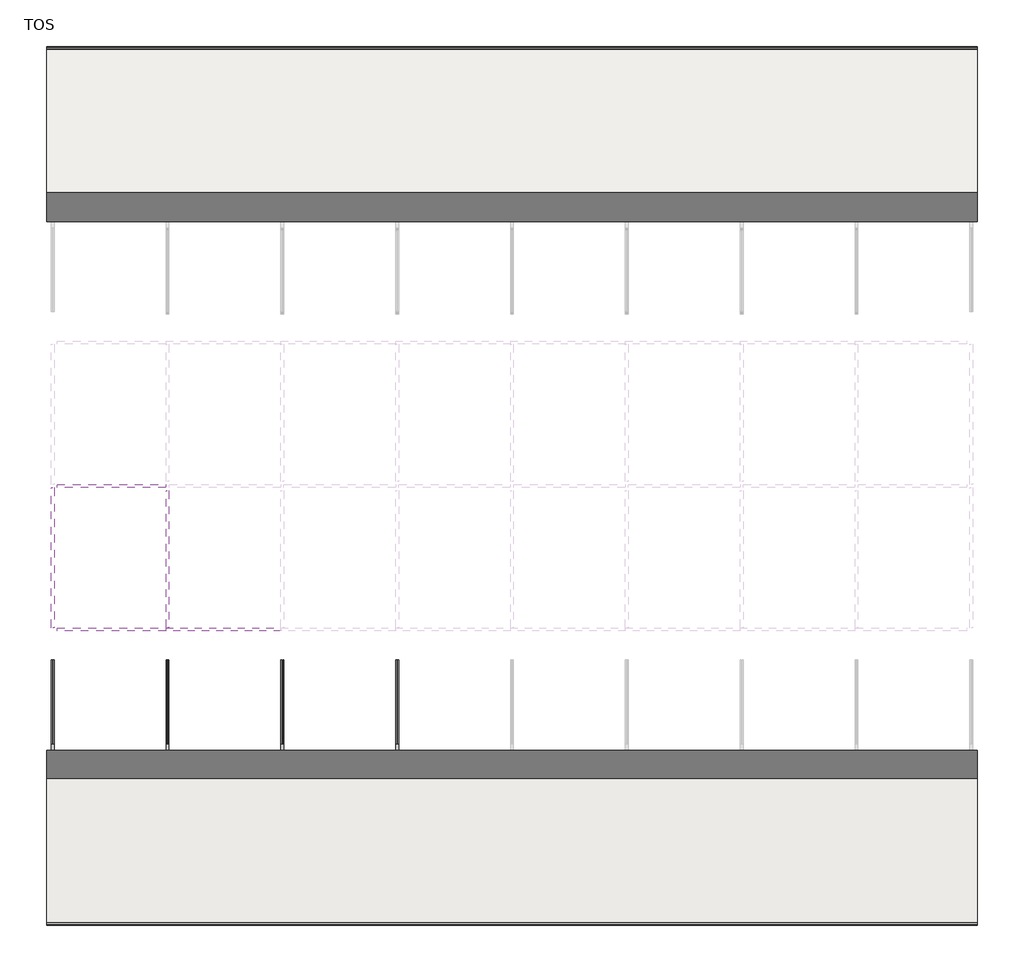
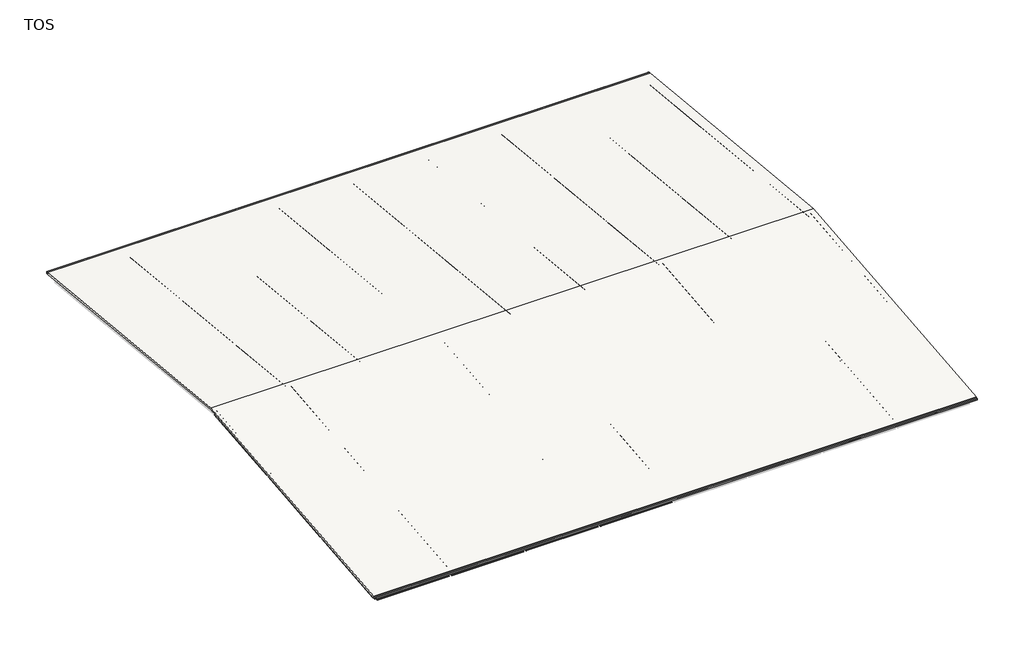
# One storey, part 1 of 5: 21 beams, 1 pipe segment, 1 roof.
"""IFC4 building model written with IfcOpenShell, lengths in millimetres."""

import ifcopenshell
import ifcopenshell.guid

model = None  # the IFC model being written
_history = None  # IfcOwnerHistory: only IFC2X3 demands one
_inside = {}  # id of a spatial element -> (the spatial element, [elements in it])
_under = {}  # id of a project, library or spatial element -> (it, [spatial elements below it])
_declared = {}  # id of a project -> (the project, [libraries it declares])
_typed = {}  # id of a type object -> (the type object, [elements of that type])
_made_of = {}  # id of a material, layer set ... -> (it, [elements and type objects made of it])


def new_model(schema):
    """Start an empty IFC model of exactly this schema.

    Asked for "IFC4X3", IfcOpenShell would pick the latest addendum, in which some entities
    have other attributes; the version numbers below select the first issue.
    IFC2X3 requires an IfcOwnerHistory on every rooted entity: one is made here for all.
    """
    global model, _history
    if schema == "IFC4X3":
        model = ifcopenshell.file(schema_version=(4, 3, 0, 0))
    else:
        model = ifcopenshell.file(schema=schema)
    _inside.clear()
    _under.clear()
    _declared.clear()
    _typed.clear()
    _made_of.clear()
    _history = None
    if model.schema == "IFC2X3":
        org = make("IfcOrganization", Name="unknown")
        user = make(
            "IfcPersonAndOrganization",
            ThePerson=make("IfcPerson", FamilyName="unknown"),
            TheOrganization=org,
        )
        app = make(
            "IfcApplication",
            ApplicationDeveloper=org,
            Version="unknown",
            ApplicationFullName="unknown",
            ApplicationIdentifier="unknown",
        )
        _history = make(
            "IfcOwnerHistory",
            OwningUser=user,
            OwningApplication=app,
            ChangeAction="ADDED",
            CreationDate=0,
        )
    return model


def make(cls, **values):
    """One entity of the class cls with the attributes given. An attribute that is None is left unset."""
    return model.create_entity(
        cls, **{name: value for name, value in values.items() if value is not None}
    )


def rooted(cls, **values):
    """An entity with a GlobalId (a new one), such as an element, a storey or a relation."""
    return make(cls, GlobalId=ifcopenshell.guid.new(), OwnerHistory=_history, **values)


def si_unit(unit_type, name, prefix=None):
    """IfcSIUnit, for example si_unit("LENGTHUNIT", "METRE", prefix="MILLI")."""
    return make("IfcSIUnit", UnitType=unit_type, Prefix=prefix, Name=name)


def assignment(units):
    """IfcUnitAssignment: the units of a project."""
    return None if units is None else make("IfcUnitAssignment", Units=units)


def point(xyz):
    """IfcCartesianPoint."""
    return None if xyz is None else make("IfcCartesianPoint", Coordinates=xyz)


def direction(xyz):
    """IfcDirection."""
    return None if xyz is None else make("IfcDirection", DirectionRatios=xyz)


def frame(location, z_axis=None, x_axis=None):
    """IfcAxis2Placement3D, a coordinate frame: its origin and axes. An axis left out is left unset."""
    return make(
        "IfcAxis2Placement3D",
        Location=point(location),
        Axis=direction(z_axis),
        RefDirection=direction(x_axis),
    )


def frame_2d(location, x_axis=None):
    """IfcAxis2Placement2D, a coordinate frame in the plane: its origin and x axis."""
    return make(
        "IfcAxis2Placement2D", Location=point(location), RefDirection=direction(x_axis)
    )


def origin():
    """The frame at (0, 0, 0) with its axes left unset."""
    return frame((0.0, 0.0, 0.0))


def place(relative_to, where):
    """IfcLocalPlacement: puts the frame where relative to a parent placement (None: the world)."""
    return make(
        "IfcLocalPlacement", PlacementRelTo=relative_to, RelativePlacement=where
    )


def context(
    kind, dimensions, precision=None, world=None, true_north=None, identifier=None
):
    """IfcGeometricRepresentationContext, for example the 3D "Model" context."""
    return make(
        "IfcGeometricRepresentationContext",
        ContextIdentifier=identifier,
        ContextType=kind,
        CoordinateSpaceDimension=dimensions,
        Precision=precision,
        WorldCoordinateSystem=world,
        TrueNorth=true_north,
    )


def project(units=None, contexts=None):
    """IfcProject with its units and contexts."""
    return rooted(
        "IfcProject",
        Name="project",
        RepresentationContexts=contexts,
        UnitsInContext=assignment(units),
    )


def spatial(cls, under=None, at=None, **own):
    """A site, building, storey or space (cls), placed at a placement, below another one or the project."""
    s = rooted(cls, ObjectPlacement=at, **own)
    if under is not None:
        _under.setdefault(under.id(), (under, []))[1].append(s)
    return s


def polyline(points):
    """IfcPolyline through the points."""
    return make("IfcPolyline", Points=[point(p) for p in points])


def circle_curve(where, radius):
    """IfcCircle in the frame where."""
    return make("IfcCircle", Position=where, Radius=radius)


def trimmed(basis, trim1, trim2, sense, master):
    """IfcTrimmedCurve: the piece of a basis curve between two trims."""
    return make(
        "IfcTrimmedCurve",
        BasisCurve=basis,
        Trim1=trim1,
        Trim2=trim2,
        SenseAgreement=sense,
        MasterRepresentation=master,
    )


def segment(curve, same_sense, transition):
    """IfcCompositeCurveSegment."""
    return make(
        "IfcCompositeCurveSegment",
        Transition=transition,
        SameSense=same_sense,
        ParentCurve=curve,
    )


def composite_curve(segments, self_intersect=None):
    """IfcCompositeCurve: segments joined end to end."""
    return make("IfcCompositeCurve", Segments=segments, SelfIntersect=self_intersect)


def outline(outer, holes=None, kind="AREA"):
    """IfcArbitraryClosedProfileDef: a profile drawn as a closed curve; with holes, ...WithVoids."""
    if holes is None:
        return make("IfcArbitraryClosedProfileDef", ProfileType=kind, OuterCurve=outer)
    return make(
        "IfcArbitraryProfileDefWithVoids",
        ProfileType=kind,
        OuterCurve=outer,
        InnerCurves=holes,
    )


def extrude(swept, where, along, depth):
    """IfcExtrudedAreaSolid: the profile swept, set in the frame where, extruded along a direction by depth."""
    return make(
        "IfcExtrudedAreaSolid",
        SweptArea=swept,
        Position=where,
        ExtrudedDirection=direction(along),
        Depth=depth,
    )


def shape(context_of_items, identifier, shape_type, items):
    """IfcShapeRepresentation: the items that make up one representation, for example the "Body"."""
    return make(
        "IfcShapeRepresentation",
        ContextOfItems=context_of_items,
        RepresentationIdentifier=identifier,
        RepresentationType=shape_type,
        Items=items,
    )


def made_of(thing, what):
    """Note that an element or type object is made of a material, layer set ...; save() writes the relation."""
    if what is not None:
        _made_of.setdefault(what.id(), (what, []))[1].append(thing)
    return thing


def element(
    cls,
    number,
    at=None,
    inside=None,
    cuts=None,
    type_object=None,
    material=None,
    context=None,
    identifier="Body",
    shape_type=None,
    held_by="IfcProductDefinitionShape",
    body=None,
    shapes=None,
    **own,
):
    """One element of the class cls, such as IfcWall. Its Tag is "e" and its number.

    at: its placement. inside: the storey or other place that contains it. cuts: it is an
    opening in that element (IfcRelVoidsElement). A single representation is given by context,
    identifier, shape_type and body (its items); several are given by shapes. held_by: the class
    of the entity that holds the representations. save() writes the other relations.
    """
    e = rooted(cls, Tag="e%d" % number, ObjectPlacement=at, **own)
    if body is not None:
        shapes = [shape(context, identifier, shape_type, body)]
    if shapes is not None:
        e.Representation = make(held_by, Representations=shapes)
    if inside is not None:
        _inside.setdefault(inside.id(), (inside, []))[1].append(e)
    if cuts is not None:
        rooted(
            "IfcRelVoidsElement", RelatingBuildingElement=cuts, RelatedOpeningElement=e
        )
    if type_object is not None:
        _typed.setdefault(type_object.id(), (type_object, []))[1].append(e)
    return made_of(e, material)


def aggregate(whole, parts):
    """IfcRelAggregates: a whole, such as a stair, and the parts it consists of."""
    return rooted("IfcRelAggregates", RelatingObject=whole, RelatedObjects=parts)


def save(model, path):
    """Write the relations noted so far, then the file.

    IfcRelAggregates (storeys below a building ...), IfcRelContainedInSpatialStructure (elements
    in a storey), IfcRelDefinesByType, IfcRelAssociatesMaterial and IfcRelDeclares: one each for
    every whole, place, type object, material and project.
    """
    for whole, parts in _under.values():
        aggregate(whole, parts)
    for where, things in _inside.values():
        rooted(
            "IfcRelContainedInSpatialStructure",
            RelatedElements=things,
            RelatingStructure=where,
        )
    for kind, things in _typed.values():
        rooted("IfcRelDefinesByType", RelatedObjects=things, RelatingType=kind)
    for what, things in _made_of.values():
        rooted("IfcRelAssociatesMaterial", RelatedObjects=things, RelatingMaterial=what)
    for by, libraries in _declared.values():
        rooted("IfcRelDeclares", RelatingContext=by, RelatedDefinitions=libraries)
    model.write(path)


model = new_model("IFC4")

# Units and contexts
model_context = context("Model", 3, world=origin())
ifc_project = project(units=[si_unit("LENGTHUNIT", "METRE", prefix="MILLI")], contexts=[model_context])

# Site, building, storey
site = spatial("IfcSite", under=ifc_project)
building = spatial("IfcBuilding", under=site)
storey = spatial("IfcBuildingStorey", under=building, Name="TOS", Elevation=9299.9618634)

# Beams
placement = place(None, origin())
element("IfcBeam", 1, ObjectType="0912_Steel Framing_H-KSD3502 : H_SB_ASB_H-600x200x11x17", at=placement, inside=storey, context=model_context, shape_type="SweptSolid", body=[
    extrude(outline(composite_curve([segment(polyline([(10599.5208589, 9716.9618634), (10599.5208589, 9699.9618634), (10399.5208589, 9699.9618634), (10399.5208589, 9716.9618634), (10472.0208589, 9716.9618634)]), True, "CONTINUOUS"), segment(trimmed(circle_curve(frame_2d((10472.0208589, 9738.9618634)), 22.0), [point((10472.0208589, 9716.9618634))], [point((10494.0208589, 9738.9618634))], True, "CARTESIAN"), True, "CONTINUOUS"), segment(polyline([(10494.0208589, 9738.9618634), (10494.0208589, 10260.9618634)]), True, "CONTINUOUS"), segment(trimmed(circle_curve(frame_2d((10472.0208589, 10260.9618634)), 22.0), [point((10494.0208589, 10260.9618634))], [point((10472.0208589, 10282.9618634))], True, "CARTESIAN"), True, "CONTINUOUS"), segment(polyline([(10472.0208589, 10282.9618634), (10399.5208589, 10282.9618634), (10399.5208589, 10299.9618634), (10599.5208589, 10299.9618634), (10599.5208589, 10282.9618634), (10527.0208589, 10282.9618634)]), True, "CONTINUOUS"), segment(trimmed(circle_curve(frame_2d((10527.0208589, 10260.9618634)), 22.0), [point((10527.0208589, 10282.9618634))], [point((10505.0208589, 10260.9618634))], True, "CARTESIAN"), True, "CONTINUOUS"), segment(polyline([(10505.0208589, 10260.9618634), (10505.0208589, 9738.9618634)]), True, "CONTINUOUS"), segment(trimmed(circle_curve(frame_2d((10527.0208589, 9738.9618634)), 22.0), [point((10505.0208589, 9738.9618634))], [point((10527.0208589, 9716.9618634))], True, "CARTESIAN"), True, "CONTINUOUS"), segment(polyline([(10527.0208589, 9716.9618634), (10599.5208589, 9716.9618634)]), True, "CONTINUOUS")], self_intersect=False)), frame((318.7, 0.0, 0.0), z_axis=(1.0, 0.0, 0.0), x_axis=(0.0, 1.0, 0.0)), (0.0, 0.0, 1.0), 7568.6),
])
element("IfcBeam", 2, ObjectType="0912_Steel Framing_H-KSD3502 : H_SB_ASB_H-600x200x11x17", at=placement, inside=storey, context=model_context, shape_type="SweptSolid", body=[
    extrude(outline(composite_curve([segment(polyline([(10599.5208589, 9716.9618634), (10599.5208589, 9699.9618634), (10399.5208589, 9699.9618634), (10399.5208589, 9716.9618634), (10472.0208589, 9716.9618634)]), True, "CONTINUOUS"), segment(trimmed(circle_curve(frame_2d((10472.0208589, 9738.9618634)), 22.0), [point((10472.0208589, 9716.9618634))], [point((10494.0208589, 9738.9618634))], True, "CARTESIAN"), True, "CONTINUOUS"), segment(polyline([(10494.0208589, 9738.9618634), (10494.0208589, 10260.9618634)]), True, "CONTINUOUS"), segment(trimmed(circle_curve(frame_2d((10472.0208589, 10260.9618634)), 22.0), [point((10494.0208589, 10260.9618634))], [point((10472.0208589, 10282.9618634))], True, "CARTESIAN"), True, "CONTINUOUS"), segment(polyline([(10472.0208589, 10282.9618634), (10399.5208589, 10282.9618634), (10399.5208589, 10299.9618634), (10599.5208589, 10299.9618634), (10599.5208589, 10282.9618634), (10527.0208589, 10282.9618634)]), True, "CONTINUOUS"), segment(trimmed(circle_curve(frame_2d((10527.0208589, 10260.9618634)), 22.0), [point((10527.0208589, 10282.9618634))], [point((10505.0208589, 10260.9618634))], True, "CARTESIAN"), True, "CONTINUOUS"), segment(polyline([(10505.0208589, 10260.9618634), (10505.0208589, 9738.9618634)]), True, "CONTINUOUS"), segment(trimmed(circle_curve(frame_2d((10527.0208589, 9738.9618634)), 22.0), [point((10505.0208589, 9738.9618634))], [point((10527.0208589, 9716.9618634))], True, "CARTESIAN"), True, "CONTINUOUS"), segment(polyline([(10527.0208589, 9716.9618634), (10599.5208589, 9716.9618634)]), True, "CONTINUOUS")], self_intersect=False)), frame((7900.0, 0.0, 0.0), z_axis=(1.0, 0.0, 0.0), x_axis=(0.0, 1.0, 0.0)), (0.0, 0.0, 1.0), 7987.3),
])
element("IfcBeam", 3, ObjectType="0912_Steel Framing_H-KSD3502 : H_SB_ASB_H-600x200x11x17", at=placement, inside=storey, context=model_context, shape_type="SweptSolid", body=[
    extrude(outline(composite_curve([segment(polyline([(10599.5208589, 9716.9618634), (10599.5208589, 9699.9618634), (10399.5208589, 9699.9618634), (10399.5208589, 9716.9618634), (10472.0208589, 9716.9618634)]), True, "CONTINUOUS"), segment(trimmed(circle_curve(frame_2d((10472.0208589, 9738.9618634)), 22.0), [point((10472.0208589, 9716.9618634))], [point((10494.0208589, 9738.9618634))], True, "CARTESIAN"), True, "CONTINUOUS"), segment(polyline([(10494.0208589, 9738.9618634), (10494.0208589, 10260.9618634)]), True, "CONTINUOUS"), segment(trimmed(circle_curve(frame_2d((10472.0208589, 10260.9618634)), 22.0), [point((10494.0208589, 10260.9618634))], [point((10472.0208589, 10282.9618634))], True, "CARTESIAN"), True, "CONTINUOUS"), segment(polyline([(10472.0208589, 10282.9618634), (10399.5208589, 10282.9618634), (10399.5208589, 10299.9618634), (10599.5208589, 10299.9618634), (10599.5208589, 10282.9618634), (10527.0208589, 10282.9618634)]), True, "CONTINUOUS"), segment(trimmed(circle_curve(frame_2d((10527.0208589, 10260.9618634)), 22.0), [point((10527.0208589, 10282.9618634))], [point((10505.0208589, 10260.9618634))], True, "CARTESIAN"), True, "CONTINUOUS"), segment(polyline([(10505.0208589, 10260.9618634), (10505.0208589, 9738.9618634)]), True, "CONTINUOUS"), segment(trimmed(circle_curve(frame_2d((10527.0208589, 9738.9618634)), 22.0), [point((10505.0208589, 9738.9618634))], [point((10527.0208589, 9716.9618634))], True, "CARTESIAN"), True, "CONTINUOUS"), segment(polyline([(10527.0208589, 9716.9618634), (10599.5208589, 9716.9618634)]), True, "CONTINUOUS")], self_intersect=False)), frame((15900.0, 0.0, 0.0), z_axis=(1.0, 0.0, 0.0), x_axis=(0.0, 1.0, 0.0)), (0.0, 0.0, 1.0), 7987.3),
])
element("IfcBeam", 4, ObjectType="0912_Steel Framing_H-KSD3502 : H_SB_ASB_H-600x200x11x17", at=placement, inside=storey, context=model_context, shape_type="SweptSolid", body=[
    extrude(outline(composite_curve([segment(polyline([(10599.5208589, 9716.9618634), (10599.5208589, 9699.9618634), (10399.5208589, 9699.9618634), (10399.5208589, 9716.9618634), (10472.0208589, 9716.9618634)]), True, "CONTINUOUS"), segment(trimmed(circle_curve(frame_2d((10472.0208589, 9738.9618634)), 22.0), [point((10472.0208589, 9716.9618634))], [point((10494.0208589, 9738.9618634))], True, "CARTESIAN"), True, "CONTINUOUS"), segment(polyline([(10494.0208589, 9738.9618634), (10494.0208589, 10260.9618634)]), True, "CONTINUOUS"), segment(trimmed(circle_curve(frame_2d((10472.0208589, 10260.9618634)), 22.0), [point((10494.0208589, 10260.9618634))], [point((10472.0208589, 10282.9618634))], True, "CARTESIAN"), True, "CONTINUOUS"), segment(polyline([(10472.0208589, 10282.9618634), (10399.5208589, 10282.9618634), (10399.5208589, 10299.9618634), (10599.5208589, 10299.9618634), (10599.5208589, 10282.9618634), (10527.0208589, 10282.9618634)]), True, "CONTINUOUS"), segment(trimmed(circle_curve(frame_2d((10527.0208589, 10260.9618634)), 22.0), [point((10527.0208589, 10282.9618634))], [point((10505.0208589, 10260.9618634))], True, "CARTESIAN"), True, "CONTINUOUS"), segment(polyline([(10505.0208589, 10260.9618634), (10505.0208589, 9738.9618634)]), True, "CONTINUOUS"), segment(trimmed(circle_curve(frame_2d((10527.0208589, 9738.9618634)), 22.0), [point((10505.0208589, 9738.9618634))], [point((10527.0208589, 9716.9618634))], True, "CARTESIAN"), True, "CONTINUOUS"), segment(polyline([(10527.0208589, 9716.9618634), (10599.5208589, 9716.9618634)]), True, "CONTINUOUS")], self_intersect=False)), frame((23900.0, 0.0, 0.0), z_axis=(1.0, 0.0, 0.0), x_axis=(0.0, 1.0, 0.0)), (0.0, 0.0, 1.0), 7987.3),
])
element("IfcBeam", 5, ObjectType="0912_Steel Framing_H-KSD3502 : H_SB_ASB_H-600x200x11x17", at=placement, inside=storey, context=model_context, shape_type="SweptSolid", body=[
    extrude(outline(composite_curve([segment(polyline([(599.5208589, 8716.9618634), (599.5208589, 8699.9618634), (399.5208589, 8699.9618634), (399.5208589, 8716.9618634), (472.0208589, 8716.9618634)]), True, "CONTINUOUS"), segment(trimmed(circle_curve(frame_2d((472.0208589, 8738.9618634)), 22.0), [point((472.0208589, 8716.9618634))], [point((494.0208589, 8738.9618634))], True, "CARTESIAN"), True, "CONTINUOUS"), segment(polyline([(494.0208589, 8738.9618634), (494.0208589, 9260.9618634)]), True, "CONTINUOUS"), segment(trimmed(circle_curve(frame_2d((472.0208589, 9260.9618634)), 22.0), [point((494.0208589, 9260.9618634))], [point((472.0208589, 9282.9618634))], True, "CARTESIAN"), True, "CONTINUOUS"), segment(polyline([(472.0208589, 9282.9618634), (399.5208589, 9282.9618634), (399.5208589, 9299.9618634), (599.5208589, 9299.9618634), (599.5208589, 9282.9618634), (527.0208589, 9282.9618634)]), True, "CONTINUOUS"), segment(trimmed(circle_curve(frame_2d((527.0208589, 9260.9618634)), 22.0), [point((527.0208589, 9282.9618634))], [point((505.0208589, 9260.9618634))], True, "CARTESIAN"), True, "CONTINUOUS"), segment(polyline([(505.0208589, 9260.9618634), (505.0208589, 8738.9618634)]), True, "CONTINUOUS"), segment(trimmed(circle_curve(frame_2d((527.0208589, 8738.9618634)), 22.0), [point((505.0208589, 8738.9618634))], [point((527.0208589, 8716.9618634))], True, "CARTESIAN"), True, "CONTINUOUS"), segment(polyline([(527.0208589, 8716.9618634), (599.5208589, 8716.9618634)]), True, "CONTINUOUS")], self_intersect=False)), frame((113.7, 0.0, 0.0), z_axis=(1.0, 0.0, 0.0), x_axis=(0.0, 1.0, 0.0)), (0.0, 0.0, 1.0), 7772.6),
])
element("IfcBeam", 6, ObjectType="0912_Steel Framing_H-KSD3502 : H_SB_ASB_H-600x200x11x17", at=placement, inside=storey, context=model_context, shape_type="SweptSolid", body=[
    extrude(outline(composite_curve([segment(polyline([(599.5208589, 8716.9618634), (599.5208589, 8699.9618634), (399.5208589, 8699.9618634), (399.5208589, 8716.9618634), (472.0208589, 8716.9618634)]), True, "CONTINUOUS"), segment(trimmed(circle_curve(frame_2d((472.0208589, 8738.9618634)), 22.0), [point((472.0208589, 8716.9618634))], [point((494.0208589, 8738.9618634))], True, "CARTESIAN"), True, "CONTINUOUS"), segment(polyline([(494.0208589, 8738.9618634), (494.0208589, 9260.9618634)]), True, "CONTINUOUS"), segment(trimmed(circle_curve(frame_2d((472.0208589, 9260.9618634)), 22.0), [point((494.0208589, 9260.9618634))], [point((472.0208589, 9282.9618634))], True, "CARTESIAN"), True, "CONTINUOUS"), segment(polyline([(472.0208589, 9282.9618634), (399.5208589, 9282.9618634), (399.5208589, 9299.9618634), (599.5208589, 9299.9618634), (599.5208589, 9282.9618634), (527.0208589, 9282.9618634)]), True, "CONTINUOUS"), segment(trimmed(circle_curve(frame_2d((527.0208589, 9260.9618634)), 22.0), [point((527.0208589, 9282.9618634))], [point((505.0208589, 9260.9618634))], True, "CARTESIAN"), True, "CONTINUOUS"), segment(polyline([(505.0208589, 9260.9618634), (505.0208589, 8738.9618634)]), True, "CONTINUOUS"), segment(trimmed(circle_curve(frame_2d((527.0208589, 8738.9618634)), 22.0), [point((505.0208589, 8738.9618634))], [point((527.0208589, 8716.9618634))], True, "CARTESIAN"), True, "CONTINUOUS"), segment(polyline([(527.0208589, 8716.9618634), (599.5208589, 8716.9618634)]), True, "CONTINUOUS")], self_intersect=False)), frame((8113.7, 0.0, 0.0), z_axis=(1.0, 0.0, 0.0), x_axis=(0.0, 1.0, 0.0)), (0.0, 0.0, 1.0), 7772.6),
])
element("IfcBeam", 7, ObjectType="0912_Steel Framing_H-KSD3502 : H_SB_ASB_H-600x200x11x17", at=placement, inside=storey, context=model_context, shape_type="SweptSolid", body=[
    extrude(outline(composite_curve([segment(polyline([(599.5208589, 8716.9618634), (599.5208589, 8699.9618634), (399.5208589, 8699.9618634), (399.5208589, 8716.9618634), (472.0208589, 8716.9618634)]), True, "CONTINUOUS"), segment(trimmed(circle_curve(frame_2d((472.0208589, 8738.9618634)), 22.0), [point((472.0208589, 8716.9618634))], [point((494.0208589, 8738.9618634))], True, "CARTESIAN"), True, "CONTINUOUS"), segment(polyline([(494.0208589, 8738.9618634), (494.0208589, 9260.9618634)]), True, "CONTINUOUS"), segment(trimmed(circle_curve(frame_2d((472.0208589, 9260.9618634)), 22.0), [point((494.0208589, 9260.9618634))], [point((472.0208589, 9282.9618634))], True, "CARTESIAN"), True, "CONTINUOUS"), segment(polyline([(472.0208589, 9282.9618634), (399.5208589, 9282.9618634), (399.5208589, 9299.9618634), (599.5208589, 9299.9618634), (599.5208589, 9282.9618634), (527.0208589, 9282.9618634)]), True, "CONTINUOUS"), segment(trimmed(circle_curve(frame_2d((527.0208589, 9260.9618634)), 22.0), [point((527.0208589, 9282.9618634))], [point((505.0208589, 9260.9618634))], True, "CARTESIAN"), True, "CONTINUOUS"), segment(polyline([(505.0208589, 9260.9618634), (505.0208589, 8738.9618634)]), True, "CONTINUOUS"), segment(trimmed(circle_curve(frame_2d((527.0208589, 8738.9618634)), 22.0), [point((505.0208589, 8738.9618634))], [point((527.0208589, 8716.9618634))], True, "CARTESIAN"), True, "CONTINUOUS"), segment(polyline([(527.0208589, 8716.9618634), (599.5208589, 8716.9618634)]), True, "CONTINUOUS")], self_intersect=False)), frame((16113.7, 0.0, 0.0), z_axis=(1.0, 0.0, 0.0), x_axis=(0.0, 1.0, 0.0)), (0.0, 0.0, 1.0), 7772.6),
])
element("IfcBeam", 8, ObjectType="0912_Steel Framing_H-KSD3502 : H_SB_ASB_H-600x200x11x17", at=placement, inside=storey, context=model_context, shape_type="SweptSolid", body=[
    extrude(outline(composite_curve([segment(polyline([(599.5208589, 8716.9618634), (599.5208589, 8699.9618634), (399.5208589, 8699.9618634), (399.5208589, 8716.9618634), (472.0208589, 8716.9618634)]), True, "CONTINUOUS"), segment(trimmed(circle_curve(frame_2d((472.0208589, 8738.9618634)), 22.0), [point((472.0208589, 8716.9618634))], [point((494.0208589, 8738.9618634))], True, "CARTESIAN"), True, "CONTINUOUS"), segment(polyline([(494.0208589, 8738.9618634), (494.0208589, 9260.9618634)]), True, "CONTINUOUS"), segment(trimmed(circle_curve(frame_2d((472.0208589, 9260.9618634)), 22.0), [point((494.0208589, 9260.9618634))], [point((472.0208589, 9282.9618634))], True, "CARTESIAN"), True, "CONTINUOUS"), segment(polyline([(472.0208589, 9282.9618634), (399.5208589, 9282.9618634), (399.5208589, 9299.9618634), (599.5208589, 9299.9618634), (599.5208589, 9282.9618634), (527.0208589, 9282.9618634)]), True, "CONTINUOUS"), segment(trimmed(circle_curve(frame_2d((527.0208589, 9260.9618634)), 22.0), [point((527.0208589, 9282.9618634))], [point((505.0208589, 9260.9618634))], True, "CARTESIAN"), True, "CONTINUOUS"), segment(polyline([(505.0208589, 9260.9618634), (505.0208589, 8738.9618634)]), True, "CONTINUOUS"), segment(trimmed(circle_curve(frame_2d((527.0208589, 8738.9618634)), 22.0), [point((505.0208589, 8738.9618634))], [point((527.0208589, 8716.9618634))], True, "CARTESIAN"), True, "CONTINUOUS"), segment(polyline([(527.0208589, 8716.9618634), (599.5208589, 8716.9618634)]), True, "CONTINUOUS")], self_intersect=False)), frame((24113.7, 0.0, 0.0), z_axis=(1.0, 0.0, 0.0), x_axis=(0.0, 1.0, 0.0)), (0.0, 0.0, 1.0), 7772.6),
])
element("IfcBeam", 9, ObjectType="0912_Steel Framing_H-KSD3502 : H_SB_ASB_H-600x200x11x17", at=placement, inside=storey, context=model_context, shape_type="SweptSolid", body=[
    extrude(outline(composite_curve([segment(polyline([(20599.5208589, 10716.9618634), (20599.5208589, 10699.9618634), (20399.5208589, 10699.9618634), (20399.5208589, 10716.9618634), (20472.0208589, 10716.9618634)]), True, "CONTINUOUS"), segment(trimmed(circle_curve(frame_2d((20472.0208589, 10738.9618634)), 22.0), [point((20472.0208589, 10716.9618634))], [point((20494.0208589, 10738.9618634))], True, "CARTESIAN"), True, "CONTINUOUS"), segment(polyline([(20494.0208589, 10738.9618634), (20494.0208589, 11260.9618634)]), True, "CONTINUOUS"), segment(trimmed(circle_curve(frame_2d((20472.0208589, 11260.9618634)), 22.0), [point((20494.0208589, 11260.9618634))], [point((20472.0208589, 11282.9618634))], True, "CARTESIAN"), True, "CONTINUOUS"), segment(polyline([(20472.0208589, 11282.9618634), (20399.5208589, 11282.9618634), (20399.5208589, 11299.9618634), (20599.5208589, 11299.9618634), (20599.5208589, 11282.9618634), (20527.0208589, 11282.9618634)]), True, "CONTINUOUS"), segment(trimmed(circle_curve(frame_2d((20527.0208589, 11260.9618634)), 22.0), [point((20527.0208589, 11282.9618634))], [point((20505.0208589, 11260.9618634))], True, "CARTESIAN"), True, "CONTINUOUS"), segment(polyline([(20505.0208589, 11260.9618634), (20505.0208589, 10738.9618634)]), True, "CONTINUOUS"), segment(trimmed(circle_curve(frame_2d((20527.0208589, 10738.9618634)), 22.0), [point((20505.0208589, 10738.9618634))], [point((20527.0208589, 10716.9618634))], True, "CARTESIAN"), True, "CONTINUOUS"), segment(polyline([(20527.0208589, 10716.9618634), (20599.5208589, 10716.9618634)]), True, "CONTINUOUS")], self_intersect=False)), frame((318.7, 0.0, 0.0), z_axis=(1.0, 0.0, 0.0), x_axis=(0.0, 1.0, 0.0)), (0.0, 0.0, 1.0), 7568.6),
])
element("IfcBeam", 10, ObjectType="0912_Steel Framing_H-KSD3502 : H_SB_ASB_H-600x200x11x17", at=placement, inside=storey, context=model_context, shape_type="SweptSolid", body=[
    extrude(outline(composite_curve([segment(polyline([(20599.5208589, 10716.9618634), (20599.5208589, 10699.9618634), (20399.5208589, 10699.9618634), (20399.5208589, 10716.9618634), (20472.0208589, 10716.9618634)]), True, "CONTINUOUS"), segment(trimmed(circle_curve(frame_2d((20472.0208589, 10738.9618634)), 22.0), [point((20472.0208589, 10716.9618634))], [point((20494.0208589, 10738.9618634))], True, "CARTESIAN"), True, "CONTINUOUS"), segment(polyline([(20494.0208589, 10738.9618634), (20494.0208589, 11260.9618634)]), True, "CONTINUOUS"), segment(trimmed(circle_curve(frame_2d((20472.0208589, 11260.9618634)), 22.0), [point((20494.0208589, 11260.9618634))], [point((20472.0208589, 11282.9618634))], True, "CARTESIAN"), True, "CONTINUOUS"), segment(polyline([(20472.0208589, 11282.9618634), (20399.5208589, 11282.9618634), (20399.5208589, 11299.9618634), (20599.5208589, 11299.9618634), (20599.5208589, 11282.9618634), (20527.0208589, 11282.9618634)]), True, "CONTINUOUS"), segment(trimmed(circle_curve(frame_2d((20527.0208589, 11260.9618634)), 22.0), [point((20527.0208589, 11282.9618634))], [point((20505.0208589, 11260.9618634))], True, "CARTESIAN"), True, "CONTINUOUS"), segment(polyline([(20505.0208589, 11260.9618634), (20505.0208589, 10738.9618634)]), True, "CONTINUOUS"), segment(trimmed(circle_curve(frame_2d((20527.0208589, 10738.9618634)), 22.0), [point((20505.0208589, 10738.9618634))], [point((20527.0208589, 10716.9618634))], True, "CARTESIAN"), True, "CONTINUOUS"), segment(polyline([(20527.0208589, 10716.9618634), (20599.5208589, 10716.9618634)]), True, "CONTINUOUS")], self_intersect=False)), frame((7900.0, 0.0, 0.0), z_axis=(1.0, 0.0, 0.0), x_axis=(0.0, 1.0, 0.0)), (0.0, 0.0, 1.0), 7987.3),
])
element("IfcBeam", 11, ObjectType="0912_Steel Framing_H-KSD3502 : H_SB_ASB_H-600x200x11x17", at=placement, inside=storey, context=model_context, shape_type="SweptSolid", body=[
    extrude(outline(composite_curve([segment(polyline([(30599.5208589, 11716.9618634), (30599.5208589, 11699.9618634), (30399.5208589, 11699.9618634), (30399.5208589, 11716.9618634), (30472.0208589, 11716.9618634)]), True, "CONTINUOUS"), segment(trimmed(circle_curve(frame_2d((30472.0208589, 11738.9618634)), 22.0), [point((30472.0208589, 11716.9618634))], [point((30494.0208589, 11738.9618634))], True, "CARTESIAN"), True, "CONTINUOUS"), segment(polyline([(30494.0208589, 11738.9618634), (30494.0208589, 12260.9618634)]), True, "CONTINUOUS"), segment(trimmed(circle_curve(frame_2d((30472.0208589, 12260.9618634)), 22.0), [point((30494.0208589, 12260.9618634))], [point((30472.0208589, 12282.9618634))], True, "CARTESIAN"), True, "CONTINUOUS"), segment(polyline([(30472.0208589, 12282.9618634), (30399.5208589, 12282.9618634), (30399.5208589, 12299.9618634), (30599.5208589, 12299.9618634), (30599.5208589, 12282.9618634), (30527.0208589, 12282.9618634)]), True, "CONTINUOUS"), segment(trimmed(circle_curve(frame_2d((30527.0208589, 12260.9618634)), 22.0), [point((30527.0208589, 12282.9618634))], [point((30505.0208589, 12260.9618634))], True, "CARTESIAN"), True, "CONTINUOUS"), segment(polyline([(30505.0208589, 12260.9618634), (30505.0208589, 11738.9618634)]), True, "CONTINUOUS"), segment(trimmed(circle_curve(frame_2d((30527.0208589, 11738.9618634)), 22.0), [point((30505.0208589, 11738.9618634))], [point((30527.0208589, 11716.9618634))], True, "CARTESIAN"), True, "CONTINUOUS"), segment(polyline([(30527.0208589, 11716.9618634), (30599.5208589, 11716.9618634)]), True, "CONTINUOUS")], self_intersect=False)), frame((318.7, 0.0, 0.0), z_axis=(1.0, 0.0, 0.0), x_axis=(0.0, 1.0, 0.0)), (0.0, 0.0, 1.0), 7567.6),
])
element("IfcBeam", 12, ObjectType="0912_Steel Framing_H-KSD3502 : H_SB_ASB_H-600x200x11x17", at=placement, inside=storey, context=model_context, shape_type="SweptSolid", body=[
    extrude(outline(composite_curve([segment(polyline([(-283.0, -100.0), (-299.9999999, -100.0), (-299.9999999, 100.0), (-283.0, 100.0), (-283.0, 27.5)]), True, "CONTINUOUS"), segment(trimmed(circle_curve(frame_2d((-261.0, 27.5)), 22.0), [point((-283.0, 27.5))], [point((-261.0, 5.5))], True, "CARTESIAN"), True, "CONTINUOUS"), segment(polyline([(-261.0, 5.5), (261.0, 5.5)]), True, "CONTINUOUS"), segment(trimmed(circle_curve(frame_2d((261.0, 27.5)), 22.0), [point((261.0, 5.5))], [point((283.0000001, 27.5))], True, "CARTESIAN"), True, "CONTINUOUS"), segment(polyline([(283.0000001, 27.5), (283.0000001, 100.0), (300.0, 100.0), (300.0, -100.0), (283.0000001, -100.0), (283.0000001, -27.5)]), True, "CONTINUOUS"), segment(trimmed(circle_curve(frame_2d((261.0, -27.5)), 22.0), [point((283.0000001, -27.5))], [point((261.0, -5.5))], True, "CARTESIAN"), True, "CONTINUOUS"), segment(polyline([(261.0, -5.5), (-261.0, -5.5)]), True, "CONTINUOUS"), segment(trimmed(circle_curve(frame_2d((-261.0, -27.5)), 22.0), [point((-261.0, -5.5))], [point((-283.0, -27.5))], True, "CARTESIAN"), True, "CONTINUOUS"), segment(polyline([(-283.0, -27.5), (-283.0, -100.0)]), True, "CONTINUOUS")], self_intersect=False)), frame((0.0, 844.9792439, 9033.0114332), z_axis=(0.0, 0.9950371902099892, 0.0995037190209989), x_axis=(0.0, -0.0995037190209989, 0.9950371902099892)), (0.0, 0.0, 1.0), 9558.4904971),
])
element("IfcBeam", 13, ObjectType="0912_Steel Framing_H-KSD3502 : H_SB_ASB_H-600x200x11x17", at=placement, inside=storey, context=model_context, shape_type="SweptSolid", body=[
    extrude(outline(composite_curve([segment(polyline([(-283.0, -100.0), (-299.9999999, -100.0), (-299.9999999, 100.0), (-283.0, 100.0), (-283.0, 27.5)]), True, "CONTINUOUS"), segment(trimmed(circle_curve(frame_2d((-261.0, 27.5)), 22.0), [point((-283.0, 27.5))], [point((-261.0, 5.5))], True, "CARTESIAN"), True, "CONTINUOUS"), segment(polyline([(-261.0, 5.5), (261.0000001, 5.5)]), True, "CONTINUOUS"), segment(trimmed(circle_curve(frame_2d((261.0000001, 27.5)), 22.0), [point((261.0000001, 5.5))], [point((283.0000001, 27.5))], True, "CARTESIAN"), True, "CONTINUOUS"), segment(polyline([(283.0000001, 27.5), (283.0000001, 100.0), (300.0, 100.0), (300.0, -100.0), (283.0000001, -100.0), (283.0000001, -27.5)]), True, "CONTINUOUS"), segment(trimmed(circle_curve(frame_2d((261.0000001, -27.5)), 22.0), [point((283.0000001, -27.5))], [point((261.0000001, -5.5))], True, "CARTESIAN"), True, "CONTINUOUS"), segment(polyline([(261.0000001, -5.5), (-261.0, -5.5)]), True, "CONTINUOUS"), segment(trimmed(circle_curve(frame_2d((-261.0, -27.5)), 22.0), [point((-261.0, -5.5))], [point((-283.0, -27.5))], True, "CARTESIAN"), True, "CONTINUOUS"), segment(polyline([(-283.0, -27.5), (-283.0, -100.0)]), True, "CONTINUOUS")], self_intersect=False)), frame((0.0, 10642.0089469, 10012.7144035), z_axis=(0.0, 0.9950371902099892, 0.09950371902099894), x_axis=(0.0, -0.09950371902099894, 0.9950371902099892)), (0.0, 0.0, 1.0), 9762.4731211),
])
element("IfcBeam", 14, ObjectType="0912_Steel Framing_H-KSD3502 : H_SB_ASB_H-600x200x11x17", at=placement, inside=storey, context=model_context, shape_type="SweptSolid", body=[
    extrude(outline(composite_curve([segment(polyline([(-283.0, -100.0), (-299.9999999, -100.0), (-299.9999999, 100.0), (-283.0, 100.0), (-283.0, 27.5)]), True, "CONTINUOUS"), segment(trimmed(circle_curve(frame_2d((-261.0, 27.5)), 22.0), [point((-283.0, 27.5))], [point((-261.0, 5.5))], True, "CARTESIAN"), True, "CONTINUOUS"), segment(polyline([(-261.0, 5.5), (261.0000001, 5.5)]), True, "CONTINUOUS"), segment(trimmed(circle_curve(frame_2d((261.0000001, 27.5)), 22.0), [point((261.0000001, 5.5))], [point((283.0000001, 27.5))], True, "CARTESIAN"), True, "CONTINUOUS"), segment(polyline([(283.0000001, 27.5), (283.0000001, 100.0), (300.0, 100.0), (300.0, -100.0), (283.0000001, -100.0), (283.0000001, -27.5)]), True, "CONTINUOUS"), segment(trimmed(circle_curve(frame_2d((261.0000001, -27.5)), 22.0), [point((283.0000001, -27.5))], [point((261.0000001, -5.5))], True, "CARTESIAN"), True, "CONTINUOUS"), segment(polyline([(261.0000001, -5.5), (-261.0, -5.5)]), True, "CONTINUOUS"), segment(trimmed(circle_curve(frame_2d((-261.0, -27.5)), 22.0), [point((-261.0, -5.5))], [point((-283.0, -27.5))], True, "CARTESIAN"), True, "CONTINUOUS"), segment(polyline([(-283.0, -27.5), (-283.0, -100.0)]), True, "CONTINUOUS")], self_intersect=False)), frame((0.0, 20642.0089469, 11012.7144035), z_axis=(0.0, 0.9950371902099892, 0.09950371902099896), x_axis=(0.0, -0.09950371902099896, 0.9950371902099892)), (0.0, 0.0, 1.0), 9762.4731211),
])
element("IfcBeam", 15, ObjectType="0912_Steel Framing_H-KSD3502 : H_SB_ASB_H-600x200x11x17", at=placement, inside=storey, context=model_context, shape_type="SweptSolid", body=[
    extrude(outline(composite_curve([segment(polyline([(-283.0, -100.0), (-299.9999999, -100.0), (-299.9999999, 100.0), (-283.0, 100.0), (-283.0, 27.5)]), True, "CONTINUOUS"), segment(trimmed(circle_curve(frame_2d((-261.0, 27.5)), 22.0), [point((-283.0, 27.5))], [point((-261.0, 5.5))], True, "CARTESIAN"), True, "CONTINUOUS"), segment(polyline([(-261.0, 5.5), (261.0, 5.5)]), True, "CONTINUOUS"), segment(trimmed(circle_curve(frame_2d((261.0, 27.5)), 22.0), [point((261.0, 5.5))], [point((283.0000001, 27.5))], True, "CARTESIAN"), True, "CONTINUOUS"), segment(polyline([(283.0000001, 27.5), (283.0000001, 100.0), (300.0, 100.0), (300.0, -100.0), (283.0000001, -100.0), (283.0000001, -27.5)]), True, "CONTINUOUS"), segment(trimmed(circle_curve(frame_2d((261.0, -27.5)), 22.0), [point((283.0000001, -27.5))], [point((261.0, -5.5))], True, "CARTESIAN"), True, "CONTINUOUS"), segment(polyline([(261.0, -5.5), (-261.0, -5.5)]), True, "CONTINUOUS"), segment(trimmed(circle_curve(frame_2d((-261.0, -27.5)), 22.0), [point((-261.0, -5.5))], [point((-283.0, -27.5))], True, "CARTESIAN"), True, "CONTINUOUS"), segment(polyline([(-283.0, -27.5), (-283.0, -100.0)]), True, "CONTINUOUS")], self_intersect=False)), frame((8000.0, 844.9792439, 9033.0114332), z_axis=(0.0, 0.9950371902099892, 0.0995037190209989), x_axis=(0.0, -0.0995037190209989, 0.9950371902099892)), (0.0, 0.0, 1.0), 9560.7882905),
])
element("IfcBeam", 16, ObjectType="0912_Steel Framing_H-KSD3502 : H_SB_ASB_H-600x200x11x17", at=placement, inside=storey, context=model_context, shape_type="SweptSolid", body=[
    extrude(outline(composite_curve([segment(polyline([(-283.0, -100.0), (-299.9999999, -100.0), (-299.9999999, 100.0), (-283.0, 100.0), (-283.0, 27.5)]), True, "CONTINUOUS"), segment(trimmed(circle_curve(frame_2d((-261.0, 27.5)), 22.0), [point((-283.0, 27.5))], [point((-261.0, 5.5))], True, "CARTESIAN"), True, "CONTINUOUS"), segment(polyline([(-261.0, 5.5), (261.0000001, 5.5)]), True, "CONTINUOUS"), segment(trimmed(circle_curve(frame_2d((261.0000001, 27.5)), 22.0), [point((261.0000001, 5.5))], [point((283.0000001, 27.5))], True, "CARTESIAN"), True, "CONTINUOUS"), segment(polyline([(283.0000001, 27.5), (283.0000001, 100.0), (300.0, 100.0), (300.0, -100.0), (283.0000001, -100.0), (283.0000001, -27.5)]), True, "CONTINUOUS"), segment(trimmed(circle_curve(frame_2d((261.0000001, -27.5)), 22.0), [point((283.0000001, -27.5))], [point((261.0000001, -5.5))], True, "CARTESIAN"), True, "CONTINUOUS"), segment(polyline([(261.0000001, -5.5), (-261.0, -5.5)]), True, "CONTINUOUS"), segment(trimmed(circle_curve(frame_2d((-261.0, -27.5)), 22.0), [point((-261.0, -5.5))], [point((-283.0, -27.5))], True, "CARTESIAN"), True, "CONTINUOUS"), segment(polyline([(-283.0, -27.5), (-283.0, -100.0)]), True, "CONTINUOUS")], self_intersect=False)), frame((8000.0, 10641.0188479, 10012.6153936), z_axis=(0.0, 0.9950371902099892, 0.09950371902099894), x_axis=(0.0, -0.09950371902099894, 0.9950371902099892)), (0.0, 0.0, 1.0), 9765.7659517),
])
element("IfcBeam", 17, ObjectType="0912_Steel Framing_H-KSD3502 : H_SB_ASB_H-600x200x11x17", at=placement, inside=storey, context=model_context, shape_type="SweptSolid", body=[
    extrude(outline(composite_curve([segment(polyline([(-283.0, -100.0), (-299.9999999, -100.0), (-299.9999999, 100.0), (-283.0, 100.0), (-283.0, 27.5)]), True, "CONTINUOUS"), segment(trimmed(circle_curve(frame_2d((-261.0, 27.5)), 22.0), [point((-283.0, 27.5))], [point((-261.0, 5.5))], True, "CARTESIAN"), True, "CONTINUOUS"), segment(polyline([(-261.0, 5.5), (261.0000001, 5.5)]), True, "CONTINUOUS"), segment(trimmed(circle_curve(frame_2d((261.0000001, 27.5)), 22.0), [point((261.0000001, 5.5))], [point((283.0000001, 27.5))], True, "CARTESIAN"), True, "CONTINUOUS"), segment(polyline([(283.0000001, 27.5), (283.0000001, 100.0), (300.0, 100.0), (300.0, -100.0), (283.0000001, -100.0), (283.0000001, -27.5)]), True, "CONTINUOUS"), segment(trimmed(circle_curve(frame_2d((261.0000001, -27.5)), 22.0), [point((283.0000001, -27.5))], [point((261.0000001, -5.5))], True, "CARTESIAN"), True, "CONTINUOUS"), segment(polyline([(261.0000001, -5.5), (-261.0, -5.5)]), True, "CONTINUOUS"), segment(trimmed(circle_curve(frame_2d((-261.0, -27.5)), 22.0), [point((-261.0, -5.5))], [point((-283.0, -27.5))], True, "CARTESIAN"), True, "CONTINUOUS"), segment(polyline([(-283.0, -27.5), (-283.0, -100.0)]), True, "CONTINUOUS")], self_intersect=False)), frame((8000.0, 20641.0188479, 11012.6153936), z_axis=(0.0, 0.9950371902099892, 0.09950371902099887), x_axis=(0.0, -0.09950371902099887, 0.9950371902099892)), (0.0, 0.0, 1.0), 9557.4457081),
])
element("IfcBeam", 18, ObjectType="0912_Steel Framing_H-KSD3502 : H_SB_ASB_H-600x200x11x17", at=placement, inside=storey, context=model_context, shape_type="SweptSolid", body=[
    extrude(outline(composite_curve([segment(polyline([(-283.0, -100.0), (-299.9999999, -100.0), (-299.9999999, 100.0), (-283.0, 100.0), (-283.0, 27.5)]), True, "CONTINUOUS"), segment(trimmed(circle_curve(frame_2d((-261.0, 27.5)), 22.0), [point((-283.0, 27.5))], [point((-261.0, 5.5))], True, "CARTESIAN"), True, "CONTINUOUS"), segment(polyline([(-261.0, 5.5), (261.0, 5.5)]), True, "CONTINUOUS"), segment(trimmed(circle_curve(frame_2d((261.0, 27.5)), 22.0), [point((261.0, 5.5))], [point((283.0000001, 27.5))], True, "CARTESIAN"), True, "CONTINUOUS"), segment(polyline([(283.0000001, 27.5), (283.0000001, 100.0), (300.0, 100.0), (300.0, -100.0), (283.0000001, -100.0), (283.0000001, -27.5)]), True, "CONTINUOUS"), segment(trimmed(circle_curve(frame_2d((261.0, -27.5)), 22.0), [point((283.0000001, -27.5))], [point((261.0, -5.5))], True, "CARTESIAN"), True, "CONTINUOUS"), segment(polyline([(261.0, -5.5), (-261.0, -5.5)]), True, "CONTINUOUS"), segment(trimmed(circle_curve(frame_2d((-261.0, -27.5)), 22.0), [point((-261.0, -5.5))], [point((-283.0, -27.5))], True, "CARTESIAN"), True, "CONTINUOUS"), segment(polyline([(-283.0, -27.5), (-283.0, -100.0)]), True, "CONTINUOUS")], self_intersect=False)), frame((16000.0, 844.9792439, 9033.0114332), z_axis=(0.0, 0.9950371902099892, 0.0995037190209989), x_axis=(0.0, -0.0995037190209989, 0.9950371902099892)), (0.0, 0.0, 1.0), 9560.7882905),
])
element("IfcBeam", 19, ObjectType="0912_Steel Framing_H-KSD3502 : H_SB_ASB_H-600x200x11x17", at=placement, inside=storey, context=model_context, shape_type="SweptSolid", body=[
    extrude(outline(composite_curve([segment(polyline([(-283.0, -100.0), (-299.9999999, -100.0), (-299.9999999, 100.0), (-283.0, 100.0), (-283.0, 27.5)]), True, "CONTINUOUS"), segment(trimmed(circle_curve(frame_2d((-261.0, 27.5)), 22.0), [point((-283.0, 27.5))], [point((-261.0, 5.5))], True, "CARTESIAN"), True, "CONTINUOUS"), segment(polyline([(-261.0, 5.5), (261.0000001, 5.5)]), True, "CONTINUOUS"), segment(trimmed(circle_curve(frame_2d((261.0000001, 27.5)), 22.0), [point((261.0000001, 5.5))], [point((283.0000001, 27.5))], True, "CARTESIAN"), True, "CONTINUOUS"), segment(polyline([(283.0000001, 27.5), (283.0000001, 100.0), (300.0, 100.0), (300.0, -100.0), (283.0000001, -100.0), (283.0000001, -27.5)]), True, "CONTINUOUS"), segment(trimmed(circle_curve(frame_2d((261.0000001, -27.5)), 22.0), [point((283.0000001, -27.5))], [point((261.0000001, -5.5))], True, "CARTESIAN"), True, "CONTINUOUS"), segment(polyline([(261.0000001, -5.5), (-261.0, -5.5)]), True, "CONTINUOUS"), segment(trimmed(circle_curve(frame_2d((-261.0, -27.5)), 22.0), [point((-261.0, -5.5))], [point((-283.0, -27.5))], True, "CARTESIAN"), True, "CONTINUOUS"), segment(polyline([(-283.0, -27.5), (-283.0, -100.0)]), True, "CONTINUOUS")], self_intersect=False)), frame((16000.0, 10641.0188479, 10012.6153936), z_axis=(0.0, 0.9950371902099892, 0.09950371902099894), x_axis=(0.0, -0.09950371902099894, 0.9950371902099892)), (0.0, 0.0, 1.0), 9765.7659517),
])
element("IfcBeam", 20, ObjectType="0912_Steel Framing_H-KSD3502 : H_SB_ASB_H-600x200x11x17", at=placement, inside=storey, context=model_context, shape_type="SweptSolid", body=[
    extrude(outline(composite_curve([segment(polyline([(-283.0, -100.0), (-299.9999999, -100.0), (-299.9999999, 100.0), (-283.0, 100.0), (-283.0, 27.5)]), True, "CONTINUOUS"), segment(trimmed(circle_curve(frame_2d((-261.0, 27.5)), 22.0), [point((-283.0, 27.5))], [point((-261.0, 5.5))], True, "CARTESIAN"), True, "CONTINUOUS"), segment(polyline([(-261.0, 5.5), (261.0, 5.5)]), True, "CONTINUOUS"), segment(trimmed(circle_curve(frame_2d((261.0, 27.5)), 22.0), [point((261.0, 5.5))], [point((283.0000001, 27.5))], True, "CARTESIAN"), True, "CONTINUOUS"), segment(polyline([(283.0000001, 27.5), (283.0000001, 100.0), (300.0, 100.0), (300.0, -100.0), (283.0000001, -100.0), (283.0000001, -27.5)]), True, "CONTINUOUS"), segment(trimmed(circle_curve(frame_2d((261.0, -27.5)), 22.0), [point((283.0000001, -27.5))], [point((261.0, -5.5))], True, "CARTESIAN"), True, "CONTINUOUS"), segment(polyline([(261.0, -5.5), (-261.0, -5.5)]), True, "CONTINUOUS"), segment(trimmed(circle_curve(frame_2d((-261.0, -27.5)), 22.0), [point((-261.0, -5.5))], [point((-283.0, -27.5))], True, "CARTESIAN"), True, "CONTINUOUS"), segment(polyline([(-283.0, -27.5), (-283.0, -100.0)]), True, "CONTINUOUS")], self_intersect=False)), frame((24000.0, 844.9792439, 9033.0114332), z_axis=(0.0, 0.9950371902099892, 0.09950371902099892), x_axis=(0.0, -0.09950371902099892, 0.9950371902099892)), (0.0, 0.0, 1.0), 9560.7882905),
])
element("IfcBeam", 21, ObjectType="0912_Steel Framing_H-KSD3502 : H_SB_ASB_H-600x200x11x17", at=placement, inside=storey, context=model_context, shape_type="SweptSolid", body=[
    extrude(outline(composite_curve([segment(polyline([(-283.0, -100.0), (-299.9999999, -100.0), (-299.9999999, 100.0), (-283.0, 100.0), (-283.0, 27.5)]), True, "CONTINUOUS"), segment(trimmed(circle_curve(frame_2d((-261.0, 27.5)), 22.0), [point((-283.0, 27.5))], [point((-261.0, 5.5))], True, "CARTESIAN"), True, "CONTINUOUS"), segment(polyline([(-261.0, 5.5), (261.0000001, 5.5)]), True, "CONTINUOUS"), segment(trimmed(circle_curve(frame_2d((261.0000001, 27.5)), 22.0), [point((261.0000001, 5.5))], [point((283.0000001, 27.5))], True, "CARTESIAN"), True, "CONTINUOUS"), segment(polyline([(283.0000001, 27.5), (283.0000001, 100.0), (300.0, 100.0), (300.0, -100.0), (283.0000001, -100.0), (283.0000001, -27.5)]), True, "CONTINUOUS"), segment(trimmed(circle_curve(frame_2d((261.0000001, -27.5)), 22.0), [point((283.0000001, -27.5))], [point((261.0000001, -5.5))], True, "CARTESIAN"), True, "CONTINUOUS"), segment(polyline([(261.0000001, -5.5), (-261.0, -5.5)]), True, "CONTINUOUS"), segment(trimmed(circle_curve(frame_2d((-261.0, -27.5)), 22.0), [point((-261.0, -5.5))], [point((-283.0, -27.5))], True, "CARTESIAN"), True, "CONTINUOUS"), segment(polyline([(-283.0, -27.5), (-283.0, -100.0)]), True, "CONTINUOUS")], self_intersect=False)), frame((24000.0, 10641.0188479, 10012.6153936), z_axis=(0.0, 0.9950371902099892, 0.09950371902099894), x_axis=(0.0, -0.09950371902099894, 0.9950371902099892)), (0.0, 0.0, 1.0), 9765.7659517),
])

# Pipe segment
element("IfcPipeSegment", 22, ObjectType="Steel Gutter_W200", at=placement, inside=storey, context=model_context, shape_type="SweptSolid", body=[
    extrude(outline(polyline([(60925.5208589, 9301.0469352), (60925.5208589, 9500.9591677), (60928.6958589, 9500.9591677), (60928.6958589, 9304.2219352), (61072.3585616, 9304.2219352), (61110.4585616, 9478.7341677), (61122.3458589, 9478.7341677), (61122.3458589, 9485.0841677), (61112.8208589, 9485.0841677), (61112.8208589, 9488.2591677), (61125.5208589, 9488.2591677), (61125.5208589, 9475.5591677), (61112.8208589, 9475.5591677), (61074.7208589, 9301.0469352), (60925.5208589, 9301.0469352)])), frame((-426.0, 0.0, 0.0), z_axis=(1.0, 0.0, 0.0), x_axis=(0.0, 1.0, 0.0)), (0.0, 0.0, 1.0), 64852.0),
    extrude(outline(polyline([(73.5208589, 9301.0469352), (-75.6791411, 9301.0469352), (-113.7791411, 9475.5591677), (-126.4791411, 9475.5591677), (-126.4791411, 9488.2591677), (-113.7791411, 9488.2591677), (-113.7791411, 9485.0841677), (-123.3041411, 9485.0841677), (-123.3041411, 9478.7341677), (-111.4168438, 9478.7341677), (-73.3168438, 9304.2219352), (70.3458589, 9304.2219352), (70.3458589, 9500.9591677), (73.5208589, 9500.9591677), (73.5208589, 9301.0469352)])), frame((-426.0, 0.0, 0.0), z_axis=(1.0, 0.0, 0.0), x_axis=(0.0, 1.0, 0.0)), (0.0, 0.0, 1.0), 64852.0),
])

# Roof
element("IfcRoof", 23, ObjectType="H_RF_AMR_Roof Panel_Steel_Mineral Wool_T200", at=placement, inside=storey, context=model_context, shape_type="SweptSolid", body=[
    extrude(outline(polyline([(73.5208589, 9500.9591677), (30499.5208589, 12543.2410422), (60925.5208589, 9500.9591677), (60925.5208589, 9299.9618634), (30499.5208589, 12342.2437378), (73.5208589, 9299.9618634), (73.5208589, 9500.9591677)])), frame((-426.0, 0.0, 0.0), z_axis=(1.0, 0.0, 0.0), x_axis=(0.0, 1.0, 0.0)), (0.0, 0.0, 1.0), 64852.0),
])

save(model, "model.ifc")

# Revit data of these elements
# Type "0912_Steel Framing_H-KSD3502 : H_SB_ASB_H-600x200x11x17"
#   Width = 20.0 cm
#   Web Thickness = 1.1 cm
#   Web Fillet = 2.2 cm
#   Warping Constant = 1930000.0 cm⁶
#   W = 0
#   Torsional Moment of Inertia = 91.3724 cm⁴
#   Section Area = 134.4 cm²
#   Plastic Modulus weak axis = 361.0 cm³
#   Plastic Modulus strong axis = 2980.0 cm³
#   Perimeter = 1.94 m²/m
#   Nominal Weight = 106.00 kgf/m
#   Moment of Inertia weak axis = 2280.00 cm⁴
#   Moment of Inertia strong axis = 77600.00 cm⁴
#   Height = 60.0 cm
#   Flange Thickness = 1.7 cm
#   Elastic Modulus weak axis = 228.0 cm³
#   Elastic Modulus strong axis = 2590.0 cm³
#   Centroid Vertical = 30.0 cm
#   Centroid Horizontal = 10.0 cm
#   Ix = 776000000
#   Length [instance default] = 1524 mm
#   Zx = 2980000
#   b = 200 mm
#   h = 600 mm
#   r = 22 mm
#   s = 11 mm
#   t = 17 mm
#   A = 0.01344 m²
#   Structural Material [instance default] = Steel, 45-345
#   Assembly Code = ""
# Type "H_RF_AMR_Roof Panel_Steel_Mineral Wool_T200"
#   Layers, outside or top first: 200 mm no material (function 4)
# Elements 1, 2, 3, 4, 5, 6, 7, 8, 9, 10, 11, 12, 13, 14, 15, 16, 17, 18, 19, 20, 21 (IfcBeam, "0912_Steel Framing_H-KSD3502 : H_SB_ASB_H-600x200x11x17")
#   Comments = ""
#   Phase Created = New Construction
#   Materials on its faces: "Steel, 45-345"
# Element 22 (IfcPipeSegment, "Steel Gutter_W200")
#   Phase Created = New Construction
#   Materials on its faces: "Default Roof"
# Element 23 (IfcRoof, "H_RF_AMR_Roof Panel_Steel_Mineral Wool_T200")
#   built-in parameter 1001705 = 41.1524 (stored number, unit not read)
#   built-in parameter 1001710 = 33615
#   Phase Created = New Construction
#   Materials on its faces: "Default Roof"
# Materials
#   "Steel, 45-345": class "Metal", colour RGB 189 187 185, transparency 0, Description = "Steel 345 MPa", Cost = 0
#   "Default Roof": class "Miscellaneous", colour RGB 80 80 80, transparency 0
